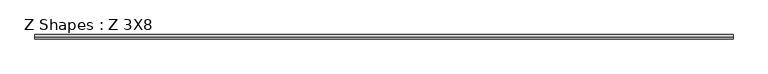
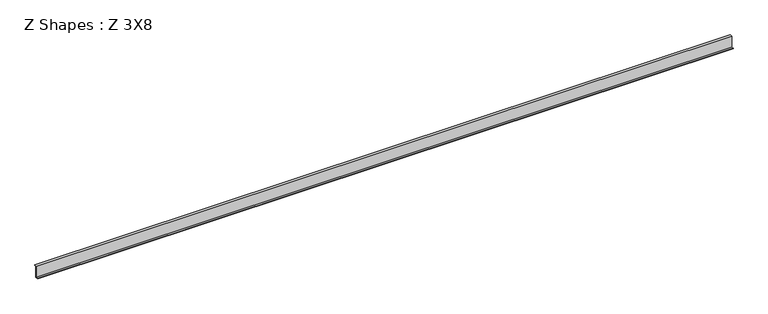
"""IFC4 building model written with IfcOpenShell, lengths in millimetres: beam geometry, Z Shapes : Z 3X8."""

from ifc_helpers import new_model, si_unit, frame, origin, place, context, project, spatial, polyline, outline, extrude, source, transform, mapped, element, save


def z_shapes_z_3x8_4b810d73(model_context):
    return source(origin(), model_context, "Body", "SweptSolid", [
        extrude(outline(polyline([(57.2805719, 92.452825), (27.1991352, 92.452825), (27.1991352, -98.809175), (-18.9194281, -98.809175), (-18.9194281, -92.459175), (19.1805719, -92.459175), (19.1805719, 102.104825), (57.2805719, 102.104825), (57.2805719, 92.452825)])), frame((-5835.65, 0.0, 0.0), z_axis=(1.0, 0.0, 0.0), x_axis=(0.0, 1.0, 0.0)), (0.0, 0.0, 1.0), 11671.2999994),
    ])


if __name__ == "__main__":
    model = new_model("IFC4")
    model_context = context("Model", 3, world=origin())
    ifc_project = project(units=[si_unit("LENGTHUNIT", "METRE", prefix="MILLI")], contexts=[model_context])
    site = spatial("IfcSite", under=ifc_project)
    building = spatial("IfcBuilding", under=site)
    placement = place(None, origin())
    z_shapes_z_3x8_shape = z_shapes_z_3x8_4b810d73(model_context)
    element("IfcBeam", 1, ObjectType="Z Shapes : Z 3X8", at=placement, inside=building, context=model_context, shape_type="MappedRepresentation", body=[
        mapped(z_shapes_z_3x8_shape, transform((0.0, 0.0, 0.0), x_axis=(1.0, 0.0, 0.0), y_axis=(0.0, 1.0, 0.0), z_axis=(0.0, 0.0, 1.0))),
    ])
    save(model, "model.ifc")

# Revit data of these elements
# Type "Z Shapes : Z 3X8"
#   Section Name Key = "W12x26"
#   Assembly Code = "B10"
#   Width = 76.2 mm
#   Web Thickness = 5.842 mm
#   Web Fillet = 7.62 mm
#   Warping Constant = 163001.3 cm⁶
#   Torsional Moment of Inertia = 12.4869 cm⁴
#   Section Area = 7.65 in²
#   Plastic Modulus weak axis = 0.00472801 (stored number, unit not read)
#   Plastic Modulus strong axis = 0.0215278 (stored number, unit not read)
#   Perimeter = 15.0571 m²/m
#   Nominal Weight = 379.441 N/m
#   Moment of Inertia weak axis = 720.08 cm⁴
#   Moment of Inertia strong axis = 8491.12 cm⁴
#   Height = 184.912 mm
#   Flange Thickness = 9.652 mm
#   Elastic Modulus weak axis = 0.00309028 (stored number, unit not read)
#   Elastic Modulus strong axis = 0.0193287 (stored number, unit not read)
#   Centroid Vertical = 92.456 mm
#   Centroid Horizontal = 38.1 mm
#   Length [instance default] = 5' - 0"
#   Structural Material [instance default] = Steel ASTM A992
#   Principal Axes Angle = 0
# Element 1 (IfcBeam, "Z Shapes : Z 3X8")
#   Structural Material = accent 2
#   Materials on its faces: "accent 2"
# Materials
#   "Steel ASTM A992": class "Metal", colour RGB 189 187 185, transparency 0, Description = "Structural steel 50ksi", Cost = 0
#   "accent 2": class "Wood", colour RGB 80 80 80, transparency 0, Description = "Wood framing, thermal airspace", Cost = 0
